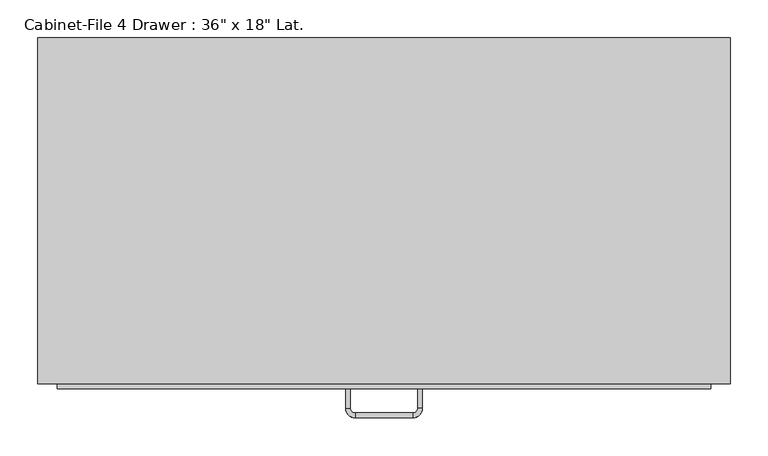
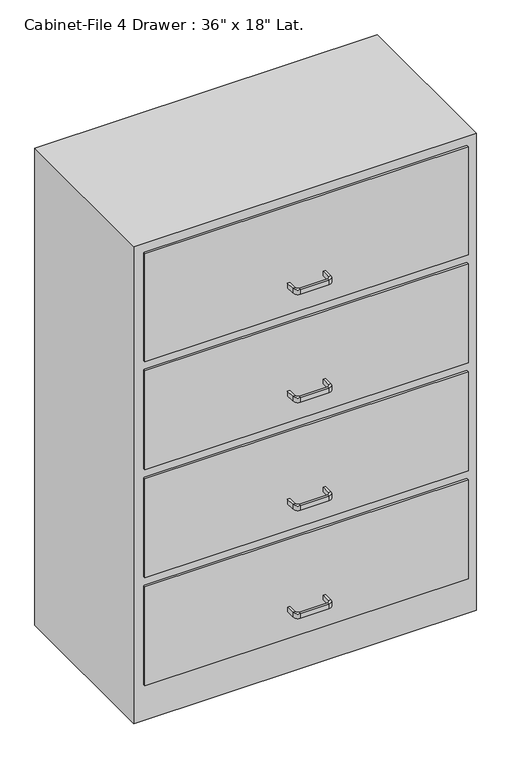
"""IFC4 building model written with IfcOpenShell, lengths in millimetres: furniture geometry."""

from ifc_helpers import new_model, si_unit, frame, origin, origin_with_axes, place, context, project, spatial, polyline, circle_curve, outline, extrude, source, transform, mapped, element, save
from ifc_brep_helpers import plane_surface, cylinder_surface, revolved_surface, advanced_brep


def furniture_7033c86c(model_context):
    return source(origin(), model_context, "Body", "SolidModel", [
        extrude(outline(polyline([(329.303553, 86.4656999), (329.303553, -370.7343001), (-585.096447, -370.7343001), (-585.096447, 86.4656999), (329.303553, 86.4656999)])), origin_with_axes(), (0.0, 0.0, 1.0), 1346.2),
        extrude(outline(polyline([(303.903553, -377.0843001), (-559.696447, -377.0843001), (-559.696447, -370.7343001), (303.903553, -370.7343001), (303.903553, -377.0843001)])), frame((0.0, 0.0, 1016.0), z_axis=(0.0, 0.0, 1.0), x_axis=(1.0, 0.0, 0.0)), (0.0, 0.0, 1.0), 304.8),
        extrude(outline(polyline([(303.903553, -377.0843001), (-559.696447, -377.0843001), (-559.696447, -370.7343001), (303.903553, -370.7343001), (303.903553, -377.0843001)])), frame((0.0, 0.0, 711.2), z_axis=(0.0, 0.0, 1.0), x_axis=(1.0, 0.0, 0.0)), (0.0, 0.0, 1.0), 279.4),
        extrude(outline(polyline([(303.903553, -377.0843001), (-559.696447, -377.0843001), (-559.696447, -370.7343001), (303.903553, -370.7343001), (303.903553, -377.0843001)])), frame((0.0, 0.0, 406.4), z_axis=(0.0, 0.0, 1.0), x_axis=(1.0, 0.0, 0.0)), (0.0, 0.0, 1.0), 279.4),
        extrude(outline(polyline([(303.903553, -377.0843001), (-559.696447, -377.0843001), (-559.696447, -370.7343001), (303.903553, -370.7343001), (303.903553, -377.0843001)])), frame((0.0, 0.0, 101.6), z_axis=(0.0, 0.0, 1.0), x_axis=(1.0, 0.0, 0.0)), (0.0, 0.0, 1.0), 279.4),
        advanced_brep(
        [(-172.346447, -377.0843001, 177.8), (-178.696447, -377.0843001, 177.8), (-178.696447, -377.0843001, 190.5), (-172.346447, -377.0843001, 190.5), (-172.346447, -402.4843001, 177.8), (-178.696447, -402.4843001, 177.8), (-178.696447, -402.4843001, 190.5), (-172.346447, -402.4843001, 190.5), (-165.996447, -415.1843001, 177.8), (-165.996447, -408.8343001, 177.8), (-165.996447, -415.1843001, 190.5), (-165.996447, -408.8343001, 190.5), (-89.796447, -408.8343001, 177.8), (-89.796447, -415.1843001, 177.8), (-89.796447, -415.1843001, 190.5), (-89.796447, -408.8343001, 190.5), (-77.096447, -402.4843001, 177.8), (-83.446447, -402.4843001, 177.8), (-77.096447, -402.4843001, 190.5), (-83.446447, -402.4843001, 190.5), (-83.446447, -377.0843001, 177.8), (-83.446447, -377.0843001, 190.5), (-77.096447, -377.0843001, 190.5), (-77.096447, -377.0843001, 177.8)],
        [
            (0, 1),
            (1, 2),
            (2, 3),
            (3, 0),
            (0, 4),
            (4, 5),
            (5, 1),
            (5, 6),
            (6, 2),
            (6, 7),
            (7, 3),
            (7, 4),
            (8, 5, circle_curve(frame((-165.996447, -402.4843001, 177.8), z_axis=(0.0, 0.0, -1.0), x_axis=(-1.0, 0.0, 0.0)), 12.7)),
            (4, 9, circle_curve(frame((-165.996447, -402.4843001, 177.8), z_axis=(0.0, 0.0, 1.0), x_axis=(-1.0, 0.0, 0.0)), 6.35)),
            (9, 8),
            (10, 6, circle_curve(frame((-165.996447, -402.4843001, 190.5), z_axis=(0.0, 0.0, -1.0), x_axis=(-1.0, 0.0, 0.0)), 12.7)),
            (8, 10),
            (11, 7, circle_curve(frame((-165.996447, -402.4843001, 190.5), z_axis=(0.0, 0.0, -1.0), x_axis=(-1.0, 0.0, 0.0)), 6.35)),
            (10, 11),
            (11, 9),
            (9, 12),
            (12, 13),
            (13, 8),
            (13, 14),
            (14, 10),
            (14, 15),
            (15, 11),
            (15, 12),
            (16, 13, circle_curve(frame((-89.796447, -402.4843001, 177.8), z_axis=(0.0, 0.0, -1.0), x_axis=(0.0, -1.0, 0.0)), 12.7)),
            (12, 17, circle_curve(frame((-89.796447, -402.4843001, 177.8), z_axis=(0.0, 0.0, 1.0), x_axis=(0.0, -1.0, 0.0)), 6.35)),
            (17, 16),
            (18, 14, circle_curve(frame((-89.796447, -402.4843001, 190.5), z_axis=(0.0, 0.0, -1.0), x_axis=(0.0, -1.0, 0.0)), 12.7)),
            (16, 18),
            (19, 15, circle_curve(frame((-89.796447, -402.4843001, 190.5), z_axis=(0.0, 0.0, -1.0), x_axis=(0.0, -1.0, 0.0)), 6.35)),
            (18, 19),
            (19, 17),
            (20, 21),
            (21, 22),
            (22, 23),
            (23, 20),
            (17, 20),
            (23, 16),
            (22, 18),
            (21, 19),
        ],
        [
            plane_surface(frame((-1283.614694, -377.0843001, 0.0), z_axis=(0.0, 1.0, 0.0), x_axis=(0.0, 0.0, -1.0))),
            plane_surface(frame((-172.346447, -377.0843001, 177.8), z_axis=(0.0, 0.0, -1.0), x_axis=(0.0, -1.0, 0.0))),
            plane_surface(frame((-178.696447, -377.0843001, 177.8), z_axis=(-1.0, 0.0, 0.0), x_axis=(0.0, -1.0, 0.0))),
            plane_surface(frame((-178.696447, -377.0843001, 190.5), z_axis=(0.0, 0.0, 1.0), x_axis=(0.0, -1.0, 0.0))),
            plane_surface(frame((-172.346447, -377.0843001, 190.5), z_axis=(1.0, 0.0, 0.0), x_axis=(0.0, -1.0, 0.0))),
            plane_surface(frame((-165.996447, -402.4843001, 177.8), z_axis=(0.0, 0.0, -1.0), x_axis=(-1.0, 0.0, 0.0))),
            cylinder_surface(frame((-165.996447, -402.4843001, 0.0), z_axis=(0.0, 0.0, 1.0), x_axis=(-1.0, 0.0, 0.0)), 12.7),
            plane_surface(frame((-165.996447, -402.4843001, 190.5), z_axis=(0.0, 0.0, 1.0), x_axis=(-1.0, 0.0, 0.0))),
            revolved_surface(polyline([(-172.34644699999998, -402.4843001, 190.5), (-172.34644699999998, -402.4843001, 177.8)]), (-165.996447, -402.4843001, 0.0), (0.0, 0.0, 1.0)),
            plane_surface(frame((-165.996447, -408.8343001, 177.8), z_axis=(0.0, 0.0, -1.0), x_axis=(1.0, 0.0, 0.0))),
            plane_surface(frame((-165.996447, -415.1843001, 177.8), z_axis=(0.0, -1.0, 0.0), x_axis=(1.0, 0.0, 0.0))),
            plane_surface(frame((-165.996447, -415.1843001, 190.5), z_axis=(0.0, 0.0, 1.0), x_axis=(1.0, 0.0, 0.0))),
            plane_surface(frame((-165.996447, -408.8343001, 190.5), z_axis=(0.0, 1.0, 0.0), x_axis=(1.0, 0.0, 0.0))),
            plane_surface(frame((-89.796447, -402.4843001, 177.8), z_axis=(0.0, 0.0, -1.0), x_axis=(0.0, -1.0, 0.0))),
            cylinder_surface(frame((-89.796447, -402.4843001, 0.0), z_axis=(0.0, 0.0, 1.0), x_axis=(0.0, -1.0, 0.0)), 12.7),
            plane_surface(frame((-89.796447, -402.4843001, 190.5), z_axis=(0.0, 0.0, 1.0), x_axis=(0.0, -1.0, 0.0))),
            revolved_surface(polyline([(-89.796447, -408.8343001, 190.5), (-89.796447, -408.8343001, 177.8)]), (-89.796447, -402.4843001, 0.0), (0.0, 0.0, 1.0)),
            plane_surface(frame((-1182.014694, -377.0843001, 0.0), z_axis=(0.0, 1.0, 0.0), x_axis=(0.0, 0.0, 1.0))),
            plane_surface(frame((-83.446447, -402.4843001, 177.8), z_axis=(0.0, 0.0, -1.0), x_axis=(0.0, 1.0, 0.0))),
            plane_surface(frame((-77.096447, -402.4843001, 177.8), z_axis=(1.0, 0.0, 0.0), x_axis=(0.0, 1.0, 0.0))),
            plane_surface(frame((-77.096447, -402.4843001, 190.5), z_axis=(0.0, 0.0, 1.0), x_axis=(0.0, 1.0, 0.0))),
            plane_surface(frame((-83.446447, -402.4843001, 190.5), z_axis=(-1.0, 0.0, 0.0), x_axis=(0.0, 1.0, 0.0))),
        ],
        [
            (0, [[1, 2, 3, 4]]),
            (1, [[-1, 5, 6, 7]]),
            (2, [[-2, -7, 8, 9]]),
            (3, [[-3, -9, 10, 11]]),
            (4, [[-4, -11, 12, -5]]),
            (5, [[13, -6, 14, 15]]),
            (6, [[16, -8, -13, 17]]),
            (7, [[18, -10, -16, 19]]),
            (8, [[-14, -12, -18, 20]]),
            (9, [[-15, 21, 22, 23]]),
            (10, [[-17, -23, 24, 25]]),
            (11, [[-19, -25, 26, 27]]),
            (12, [[-20, -27, 28, -21]]),
            (13, [[29, -22, 30, 31]]),
            (14, [[32, -24, -29, 33]]),
            (15, [[34, -26, -32, 35]]),
            (16, [[-30, -28, -34, 36]]),
            (17, [[37, 38, 39, 40]]),
            (18, [[-31, 41, -40, 42]]),
            (19, [[-33, -42, -39, 43]]),
            (20, [[-35, -43, -38, 44]]),
            (21, [[-36, -44, -37, -41]]),
        ],
    ),
        advanced_brep(
        [(-172.346447, -377.0843001, 482.6), (-178.696447, -377.0843001, 482.6), (-178.696447, -377.0843001, 495.3), (-172.346447, -377.0843001, 495.3), (-172.346447, -402.4843001, 482.6), (-178.696447, -402.4843001, 482.6), (-178.696447, -402.4843001, 495.3), (-172.346447, -402.4843001, 495.3), (-165.996447, -415.1843001, 482.6), (-165.996447, -408.8343001, 482.6), (-165.996447, -415.1843001, 495.3), (-165.996447, -408.8343001, 495.3), (-89.796447, -408.8343001, 482.6), (-89.796447, -415.1843001, 482.6), (-89.796447, -415.1843001, 495.3), (-89.796447, -408.8343001, 495.3), (-77.096447, -402.4843001, 482.6), (-83.446447, -402.4843001, 482.6), (-77.096447, -402.4843001, 495.3), (-83.446447, -402.4843001, 495.3), (-83.446447, -377.0843001, 482.6), (-83.446447, -377.0843001, 495.3), (-77.096447, -377.0843001, 495.3), (-77.096447, -377.0843001, 482.6)],
        [
            (0, 1),
            (1, 2),
            (2, 3),
            (3, 0),
            (0, 4),
            (4, 5),
            (5, 1),
            (5, 6),
            (6, 2),
            (6, 7),
            (7, 3),
            (7, 4),
            (8, 5, circle_curve(frame((-165.996447, -402.4843001, 482.6), z_axis=(0.0, 0.0, -1.0), x_axis=(-1.0, 0.0, 0.0)), 12.7)),
            (4, 9, circle_curve(frame((-165.996447, -402.4843001, 482.6), z_axis=(0.0, 0.0, 1.0), x_axis=(-1.0, 0.0, 0.0)), 6.35)),
            (9, 8),
            (10, 6, circle_curve(frame((-165.996447, -402.4843001, 495.3), z_axis=(0.0, 0.0, -1.0), x_axis=(-1.0, 0.0, 0.0)), 12.7)),
            (8, 10),
            (11, 7, circle_curve(frame((-165.996447, -402.4843001, 495.3), z_axis=(0.0, 0.0, -1.0), x_axis=(-1.0, 0.0, 0.0)), 6.35)),
            (10, 11),
            (11, 9),
            (9, 12),
            (12, 13),
            (13, 8),
            (13, 14),
            (14, 10),
            (14, 15),
            (15, 11),
            (15, 12),
            (16, 13, circle_curve(frame((-89.796447, -402.4843001, 482.6), z_axis=(0.0, 0.0, -1.0), x_axis=(0.0, -1.0, 0.0)), 12.7)),
            (12, 17, circle_curve(frame((-89.796447, -402.4843001, 482.6), z_axis=(0.0, 0.0, 1.0), x_axis=(0.0, -1.0, 0.0)), 6.35)),
            (17, 16),
            (18, 14, circle_curve(frame((-89.796447, -402.4843001, 495.3), z_axis=(0.0, 0.0, -1.0), x_axis=(0.0, -1.0, 0.0)), 12.7)),
            (16, 18),
            (19, 15, circle_curve(frame((-89.796447, -402.4843001, 495.3), z_axis=(0.0, 0.0, -1.0), x_axis=(0.0, -1.0, 0.0)), 6.35)),
            (18, 19),
            (19, 17),
            (20, 21),
            (21, 22),
            (22, 23),
            (23, 20),
            (17, 20),
            (23, 16),
            (22, 18),
            (21, 19),
        ],
        [
            plane_surface(frame((-1283.614694, -377.0843001, 0.0), z_axis=(0.0, 1.0, 0.0), x_axis=(0.0, 0.0, -1.0))),
            plane_surface(frame((-172.346447, -377.0843001, 482.6), z_axis=(0.0, 0.0, -1.0), x_axis=(0.0, -1.0, 0.0))),
            plane_surface(frame((-178.696447, -377.0843001, 482.6), z_axis=(-1.0, 0.0, 0.0), x_axis=(0.0, -1.0, 0.0))),
            plane_surface(frame((-178.696447, -377.0843001, 495.3), z_axis=(0.0, 0.0, 1.0), x_axis=(0.0, -1.0, 0.0))),
            plane_surface(frame((-172.346447, -377.0843001, 495.3), z_axis=(1.0, 0.0, 0.0), x_axis=(0.0, -1.0, 0.0))),
            plane_surface(frame((-165.996447, -402.4843001, 482.6), z_axis=(0.0, 0.0, -1.0), x_axis=(-1.0, 0.0, 0.0))),
            cylinder_surface(frame((-165.996447, -402.4843001, 0.0), z_axis=(0.0, 0.0, 1.0), x_axis=(-1.0, 0.0, 0.0)), 12.7),
            plane_surface(frame((-165.996447, -402.4843001, 495.3), z_axis=(0.0, 0.0, 1.0), x_axis=(-1.0, 0.0, 0.0))),
            revolved_surface(polyline([(-172.34644699999998, -402.4843001, 495.3), (-172.34644699999998, -402.4843001, 482.6)]), (-165.996447, -402.4843001, 0.0), (0.0, 0.0, 1.0)),
            plane_surface(frame((-165.996447, -408.8343001, 482.6), z_axis=(0.0, 0.0, -1.0), x_axis=(1.0, 0.0, 0.0))),
            plane_surface(frame((-165.996447, -415.1843001, 482.6), z_axis=(0.0, -1.0, 0.0), x_axis=(1.0, 0.0, 0.0))),
            plane_surface(frame((-165.996447, -415.1843001, 495.3), z_axis=(0.0, 0.0, 1.0), x_axis=(1.0, 0.0, 0.0))),
            plane_surface(frame((-165.996447, -408.8343001, 495.3), z_axis=(0.0, 1.0, 0.0), x_axis=(1.0, 0.0, 0.0))),
            plane_surface(frame((-89.796447, -402.4843001, 482.6), z_axis=(0.0, 0.0, -1.0), x_axis=(0.0, -1.0, 0.0))),
            cylinder_surface(frame((-89.796447, -402.4843001, 0.0), z_axis=(0.0, 0.0, 1.0), x_axis=(0.0, -1.0, 0.0)), 12.7),
            plane_surface(frame((-89.796447, -402.4843001, 495.3), z_axis=(0.0, 0.0, 1.0), x_axis=(0.0, -1.0, 0.0))),
            revolved_surface(polyline([(-89.796447, -408.8343001, 495.3), (-89.796447, -408.8343001, 482.6)]), (-89.796447, -402.4843001, 0.0), (0.0, 0.0, 1.0)),
            plane_surface(frame((-1182.014694, -377.0843001, 0.0), z_axis=(0.0, 1.0, 0.0), x_axis=(0.0, 0.0, 1.0))),
            plane_surface(frame((-83.446447, -402.4843001, 482.6), z_axis=(0.0, 0.0, -1.0), x_axis=(0.0, 1.0, 0.0))),
            plane_surface(frame((-77.096447, -402.4843001, 482.6), z_axis=(1.0, 0.0, 0.0), x_axis=(0.0, 1.0, 0.0))),
            plane_surface(frame((-77.096447, -402.4843001, 495.3), z_axis=(0.0, 0.0, 1.0), x_axis=(0.0, 1.0, 0.0))),
            plane_surface(frame((-83.446447, -402.4843001, 495.3), z_axis=(-1.0, 0.0, 0.0), x_axis=(0.0, 1.0, 0.0))),
        ],
        [
            (0, [[1, 2, 3, 4]]),
            (1, [[-1, 5, 6, 7]]),
            (2, [[-2, -7, 8, 9]]),
            (3, [[-3, -9, 10, 11]]),
            (4, [[-4, -11, 12, -5]]),
            (5, [[13, -6, 14, 15]]),
            (6, [[16, -8, -13, 17]]),
            (7, [[18, -10, -16, 19]]),
            (8, [[-14, -12, -18, 20]]),
            (9, [[-15, 21, 22, 23]]),
            (10, [[-17, -23, 24, 25]]),
            (11, [[-19, -25, 26, 27]]),
            (12, [[-20, -27, 28, -21]]),
            (13, [[29, -22, 30, 31]]),
            (14, [[32, -24, -29, 33]]),
            (15, [[34, -26, -32, 35]]),
            (16, [[-30, -28, -34, 36]]),
            (17, [[37, 38, 39, 40]]),
            (18, [[-31, 41, -40, 42]]),
            (19, [[-33, -42, -39, 43]]),
            (20, [[-35, -43, -38, 44]]),
            (21, [[-36, -44, -37, -41]]),
        ],
    ),
        advanced_brep(
        [(-172.346447, -377.0843001, 787.4), (-178.696447, -377.0843001, 787.4), (-178.696447, -377.0843001, 800.1), (-172.346447, -377.0843001, 800.1), (-172.346447, -402.4843001, 787.4), (-178.696447, -402.4843001, 787.4), (-178.696447, -402.4843001, 800.1), (-172.346447, -402.4843001, 800.1), (-165.996447, -415.1843001, 787.4), (-165.996447, -408.8343001, 787.4), (-165.996447, -415.1843001, 800.1), (-165.996447, -408.8343001, 800.1), (-89.796447, -408.8343001, 787.4), (-89.796447, -415.1843001, 787.4), (-89.796447, -415.1843001, 800.1), (-89.796447, -408.8343001, 800.1), (-77.096447, -402.4843001, 787.4), (-83.446447, -402.4843001, 787.4), (-77.096447, -402.4843001, 800.1), (-83.446447, -402.4843001, 800.1), (-83.446447, -377.0843001, 787.4), (-83.446447, -377.0843001, 800.1), (-77.096447, -377.0843001, 800.1), (-77.096447, -377.0843001, 787.4)],
        [
            (0, 1),
            (1, 2),
            (2, 3),
            (3, 0),
            (0, 4),
            (4, 5),
            (5, 1),
            (5, 6),
            (6, 2),
            (6, 7),
            (7, 3),
            (7, 4),
            (8, 5, circle_curve(frame((-165.996447, -402.4843001, 787.4), z_axis=(0.0, 0.0, -1.0), x_axis=(-1.0, 0.0, 0.0)), 12.7)),
            (4, 9, circle_curve(frame((-165.996447, -402.4843001, 787.4), z_axis=(0.0, 0.0, 1.0), x_axis=(-1.0, 0.0, 0.0)), 6.35)),
            (9, 8),
            (10, 6, circle_curve(frame((-165.996447, -402.4843001, 800.1), z_axis=(0.0, 0.0, -1.0), x_axis=(-1.0, 0.0, 0.0)), 12.7)),
            (8, 10),
            (11, 7, circle_curve(frame((-165.996447, -402.4843001, 800.1), z_axis=(0.0, 0.0, -1.0), x_axis=(-1.0, 0.0, 0.0)), 6.35)),
            (10, 11),
            (11, 9),
            (9, 12),
            (12, 13),
            (13, 8),
            (13, 14),
            (14, 10),
            (14, 15),
            (15, 11),
            (15, 12),
            (16, 13, circle_curve(frame((-89.796447, -402.4843001, 787.4), z_axis=(0.0, 0.0, -1.0), x_axis=(0.0, -1.0, 0.0)), 12.7)),
            (12, 17, circle_curve(frame((-89.796447, -402.4843001, 787.4), z_axis=(0.0, 0.0, 1.0), x_axis=(0.0, -1.0, 0.0)), 6.35)),
            (17, 16),
            (18, 14, circle_curve(frame((-89.796447, -402.4843001, 800.1), z_axis=(0.0, 0.0, -1.0), x_axis=(0.0, -1.0, 0.0)), 12.7)),
            (16, 18),
            (19, 15, circle_curve(frame((-89.796447, -402.4843001, 800.1), z_axis=(0.0, 0.0, -1.0), x_axis=(0.0, -1.0, 0.0)), 6.35)),
            (18, 19),
            (19, 17),
            (20, 21),
            (21, 22),
            (22, 23),
            (23, 20),
            (17, 20),
            (23, 16),
            (22, 18),
            (21, 19),
        ],
        [
            plane_surface(frame((-1283.614694, -377.0843001, 0.0), z_axis=(0.0, 1.0, 0.0), x_axis=(0.0, 0.0, -1.0))),
            plane_surface(frame((-172.346447, -377.0843001, 787.4), z_axis=(0.0, 0.0, -1.0), x_axis=(0.0, -1.0, 0.0))),
            plane_surface(frame((-178.696447, -377.0843001, 787.4), z_axis=(-1.0, 0.0, 0.0), x_axis=(0.0, -1.0, 0.0))),
            plane_surface(frame((-178.696447, -377.0843001, 800.1), z_axis=(0.0, 0.0, 1.0), x_axis=(0.0, -1.0, 0.0))),
            plane_surface(frame((-172.346447, -377.0843001, 800.1), z_axis=(1.0, 0.0, 0.0), x_axis=(0.0, -1.0, 0.0))),
            plane_surface(frame((-165.996447, -402.4843001, 787.4), z_axis=(0.0, 0.0, -1.0), x_axis=(-1.0, 0.0, 0.0))),
            cylinder_surface(frame((-165.996447, -402.4843001, 0.0), z_axis=(0.0, 0.0, 1.0), x_axis=(-1.0, 0.0, 0.0)), 12.7),
            plane_surface(frame((-165.996447, -402.4843001, 800.1), z_axis=(0.0, 0.0, 1.0), x_axis=(-1.0, 0.0, 0.0))),
            revolved_surface(polyline([(-172.34644699999998, -402.4843001, 800.1), (-172.34644699999998, -402.4843001, 787.4)]), (-165.996447, -402.4843001, 0.0), (0.0, 0.0, 1.0)),
            plane_surface(frame((-165.996447, -408.8343001, 787.4), z_axis=(0.0, 0.0, -1.0), x_axis=(1.0, 0.0, 0.0))),
            plane_surface(frame((-165.996447, -415.1843001, 787.4), z_axis=(0.0, -1.0, 0.0), x_axis=(1.0, 0.0, 0.0))),
            plane_surface(frame((-165.996447, -415.1843001, 800.1), z_axis=(0.0, 0.0, 1.0), x_axis=(1.0, 0.0, 0.0))),
            plane_surface(frame((-165.996447, -408.8343001, 800.1), z_axis=(0.0, 1.0, 0.0), x_axis=(1.0, 0.0, 0.0))),
            plane_surface(frame((-89.796447, -402.4843001, 787.4), z_axis=(0.0, 0.0, -1.0), x_axis=(0.0, -1.0, 0.0))),
            cylinder_surface(frame((-89.796447, -402.4843001, 0.0), z_axis=(0.0, 0.0, 1.0), x_axis=(0.0, -1.0, 0.0)), 12.7),
            plane_surface(frame((-89.796447, -402.4843001, 800.1), z_axis=(0.0, 0.0, 1.0), x_axis=(0.0, -1.0, 0.0))),
            revolved_surface(polyline([(-89.796447, -408.8343001, 800.1), (-89.796447, -408.8343001, 787.4)]), (-89.796447, -402.4843001, 0.0), (0.0, 0.0, 1.0)),
            plane_surface(frame((-1182.014694, -377.0843001, 0.0), z_axis=(0.0, 1.0, 0.0), x_axis=(0.0, 0.0, 1.0))),
            plane_surface(frame((-83.446447, -402.4843001, 787.4), z_axis=(0.0, 0.0, -1.0), x_axis=(0.0, 1.0, 0.0))),
            plane_surface(frame((-77.096447, -402.4843001, 787.4), z_axis=(1.0, 0.0, 0.0), x_axis=(0.0, 1.0, 0.0))),
            plane_surface(frame((-77.096447, -402.4843001, 800.1), z_axis=(0.0, 0.0, 1.0), x_axis=(0.0, 1.0, 0.0))),
            plane_surface(frame((-83.446447, -402.4843001, 800.1), z_axis=(-1.0, 0.0, 0.0), x_axis=(0.0, 1.0, 0.0))),
        ],
        [
            (0, [[1, 2, 3, 4]]),
            (1, [[-1, 5, 6, 7]]),
            (2, [[-2, -7, 8, 9]]),
            (3, [[-3, -9, 10, 11]]),
            (4, [[-4, -11, 12, -5]]),
            (5, [[13, -6, 14, 15]]),
            (6, [[16, -8, -13, 17]]),
            (7, [[18, -10, -16, 19]]),
            (8, [[-14, -12, -18, 20]]),
            (9, [[-15, 21, 22, 23]]),
            (10, [[-17, -23, 24, 25]]),
            (11, [[-19, -25, 26, 27]]),
            (12, [[-20, -27, 28, -21]]),
            (13, [[29, -22, 30, 31]]),
            (14, [[32, -24, -29, 33]]),
            (15, [[34, -26, -32, 35]]),
            (16, [[-30, -28, -34, 36]]),
            (17, [[37, 38, 39, 40]]),
            (18, [[-31, 41, -40, 42]]),
            (19, [[-33, -42, -39, 43]]),
            (20, [[-35, -43, -38, 44]]),
            (21, [[-36, -44, -37, -41]]),
        ],
    ),
        advanced_brep(
        [(-172.346447, -377.0843001, 1092.2), (-178.696447, -377.0843001, 1092.2), (-178.696447, -377.0843001, 1104.9), (-172.346447, -377.0843001, 1104.9), (-172.346447, -402.4843001, 1092.2), (-178.696447, -402.4843001, 1092.2), (-178.696447, -402.4843001, 1104.9), (-172.346447, -402.4843001, 1104.9), (-165.996447, -415.1843001, 1092.2), (-165.996447, -408.8343001, 1092.2), (-165.996447, -415.1843001, 1104.9), (-165.996447, -408.8343001, 1104.9), (-89.796447, -408.8343001, 1092.2), (-89.796447, -415.1843001, 1092.2), (-89.796447, -415.1843001, 1104.9), (-89.796447, -408.8343001, 1104.9), (-77.096447, -402.4843001, 1092.2), (-83.446447, -402.4843001, 1092.2), (-77.096447, -402.4843001, 1104.9), (-83.446447, -402.4843001, 1104.9), (-83.446447, -377.0843001, 1092.2), (-83.446447, -377.0843001, 1104.9), (-77.096447, -377.0843001, 1104.9), (-77.096447, -377.0843001, 1092.2)],
        [
            (0, 1),
            (1, 2),
            (2, 3),
            (3, 0),
            (0, 4),
            (4, 5),
            (5, 1),
            (5, 6),
            (6, 2),
            (6, 7),
            (7, 3),
            (7, 4),
            (8, 5, circle_curve(frame((-165.996447, -402.4843001, 1092.2), z_axis=(0.0, 0.0, -1.0), x_axis=(-1.0, 0.0, 0.0)), 12.7)),
            (4, 9, circle_curve(frame((-165.996447, -402.4843001, 1092.2), z_axis=(0.0, 0.0, 1.0), x_axis=(-1.0, 0.0, 0.0)), 6.35)),
            (9, 8),
            (10, 6, circle_curve(frame((-165.996447, -402.4843001, 1104.9), z_axis=(0.0, 0.0, -1.0), x_axis=(-1.0, 0.0, 0.0)), 12.7)),
            (8, 10),
            (11, 7, circle_curve(frame((-165.996447, -402.4843001, 1104.9), z_axis=(0.0, 0.0, -1.0), x_axis=(-1.0, 0.0, 0.0)), 6.35)),
            (10, 11),
            (11, 9),
            (9, 12),
            (12, 13),
            (13, 8),
            (13, 14),
            (14, 10),
            (14, 15),
            (15, 11),
            (15, 12),
            (16, 13, circle_curve(frame((-89.796447, -402.4843001, 1092.2), z_axis=(0.0, 0.0, -1.0), x_axis=(0.0, -1.0, 0.0)), 12.7)),
            (12, 17, circle_curve(frame((-89.796447, -402.4843001, 1092.2), z_axis=(0.0, 0.0, 1.0), x_axis=(0.0, -1.0, 0.0)), 6.35)),
            (17, 16),
            (18, 14, circle_curve(frame((-89.796447, -402.4843001, 1104.9), z_axis=(0.0, 0.0, -1.0), x_axis=(0.0, -1.0, 0.0)), 12.7)),
            (16, 18),
            (19, 15, circle_curve(frame((-89.796447, -402.4843001, 1104.9), z_axis=(0.0, 0.0, -1.0), x_axis=(0.0, -1.0, 0.0)), 6.35)),
            (18, 19),
            (19, 17),
            (20, 21),
            (21, 22),
            (22, 23),
            (23, 20),
            (17, 20),
            (23, 16),
            (22, 18),
            (21, 19),
        ],
        [
            plane_surface(frame((-1283.614694, -377.0843001, 0.0), z_axis=(0.0, 1.0, 0.0), x_axis=(0.0, 0.0, -1.0))),
            plane_surface(frame((-172.346447, -377.0843001, 1092.2), z_axis=(0.0, 0.0, -1.0), x_axis=(0.0, -1.0, 0.0))),
            plane_surface(frame((-178.696447, -377.0843001, 1092.2), z_axis=(-1.0, 0.0, 0.0), x_axis=(0.0, -1.0, 0.0))),
            plane_surface(frame((-178.696447, -377.0843001, 1104.9), z_axis=(0.0, 0.0, 1.0), x_axis=(0.0, -1.0, 0.0))),
            plane_surface(frame((-172.346447, -377.0843001, 1104.9), z_axis=(1.0, 0.0, 0.0), x_axis=(0.0, -1.0, 0.0))),
            plane_surface(frame((-165.996447, -402.4843001, 1092.2), z_axis=(0.0, 0.0, -1.0), x_axis=(-1.0, 0.0, 0.0))),
            cylinder_surface(frame((-165.996447, -402.4843001, 0.0), z_axis=(0.0, 0.0, 1.0), x_axis=(-1.0, 0.0, 0.0)), 12.7),
            plane_surface(frame((-165.996447, -402.4843001, 1104.9), z_axis=(0.0, 0.0, 1.0), x_axis=(-1.0, 0.0, 0.0))),
            revolved_surface(polyline([(-172.34644699999998, -402.4843001, 1104.9), (-172.34644699999998, -402.4843001, 1092.2)]), (-165.996447, -402.4843001, 0.0), (0.0, 0.0, 1.0)),
            plane_surface(frame((-165.996447, -408.8343001, 1092.2), z_axis=(0.0, 0.0, -1.0), x_axis=(1.0, 0.0, 0.0))),
            plane_surface(frame((-165.996447, -415.1843001, 1092.2), z_axis=(0.0, -1.0, 0.0), x_axis=(1.0, 0.0, 0.0))),
            plane_surface(frame((-165.996447, -415.1843001, 1104.9), z_axis=(0.0, 0.0, 1.0), x_axis=(1.0, 0.0, 0.0))),
            plane_surface(frame((-165.996447, -408.8343001, 1104.9), z_axis=(0.0, 1.0, 0.0), x_axis=(1.0, 0.0, 0.0))),
            plane_surface(frame((-89.796447, -402.4843001, 1092.2), z_axis=(0.0, 0.0, -1.0), x_axis=(0.0, -1.0, 0.0))),
            cylinder_surface(frame((-89.796447, -402.4843001, 0.0), z_axis=(0.0, 0.0, 1.0), x_axis=(0.0, -1.0, 0.0)), 12.7),
            plane_surface(frame((-89.796447, -402.4843001, 1104.9), z_axis=(0.0, 0.0, 1.0), x_axis=(0.0, -1.0, 0.0))),
            revolved_surface(polyline([(-89.796447, -408.8343001, 1104.9), (-89.796447, -408.8343001, 1092.2)]), (-89.796447, -402.4843001, 0.0), (0.0, 0.0, 1.0)),
            plane_surface(frame((-1182.014694, -377.0843001, 0.0), z_axis=(0.0, 1.0, 0.0), x_axis=(0.0, 0.0, 1.0))),
            plane_surface(frame((-83.446447, -402.4843001, 1092.2), z_axis=(0.0, 0.0, -1.0), x_axis=(0.0, 1.0, 0.0))),
            plane_surface(frame((-77.096447, -402.4843001, 1092.2), z_axis=(1.0, 0.0, 0.0), x_axis=(0.0, 1.0, 0.0))),
            plane_surface(frame((-77.096447, -402.4843001, 1104.9), z_axis=(0.0, 0.0, 1.0), x_axis=(0.0, 1.0, 0.0))),
            plane_surface(frame((-83.446447, -402.4843001, 1104.9), z_axis=(-1.0, 0.0, 0.0), x_axis=(0.0, 1.0, 0.0))),
        ],
        [
            (0, [[1, 2, 3, 4]]),
            (1, [[-1, 5, 6, 7]]),
            (2, [[-2, -7, 8, 9]]),
            (3, [[-3, -9, 10, 11]]),
            (4, [[-4, -11, 12, -5]]),
            (5, [[13, -6, 14, 15]]),
            (6, [[16, -8, -13, 17]]),
            (7, [[18, -10, -16, 19]]),
            (8, [[-14, -12, -18, 20]]),
            (9, [[-15, 21, 22, 23]]),
            (10, [[-17, -23, 24, 25]]),
            (11, [[-19, -25, 26, 27]]),
            (12, [[-20, -27, 28, -21]]),
            (13, [[29, -22, 30, 31]]),
            (14, [[32, -24, -29, 33]]),
            (15, [[34, -26, -32, 35]]),
            (16, [[-30, -28, -34, 36]]),
            (17, [[37, 38, 39, 40]]),
            (18, [[-31, 41, -40, 42]]),
            (19, [[-33, -42, -39, 43]]),
            (20, [[-35, -43, -38, 44]]),
            (21, [[-36, -44, -37, -41]]),
        ],
    ),
    ])


if __name__ == "__main__":
    model = new_model("IFC4")
    model_context = context("Model", 3, world=origin())
    ifc_project = project(units=[si_unit("LENGTHUNIT", "METRE", prefix="MILLI")], contexts=[model_context])
    site = spatial("IfcSite", under=ifc_project)
    building = spatial("IfcBuilding", under=site)
    placement = place(None, origin())
    furniture_shape = furniture_7033c86c(model_context)
    element("IfcFurniture", 1, ObjectType="Cabinet-File 4 Drawer : 36\" x 18\" Lat.", at=placement, inside=building, context=model_context, shape_type="MappedRepresentation", body=[
        mapped(furniture_shape, transform((0.0, 0.0, 0.0), x_axis=(1.0, 0.0, 0.0), y_axis=(0.0, 1.0, 0.0), z_axis=(0.0, 0.0, 1.0))),
    ])
    save(model, "model.ifc")

# Revit data of these elements
# Type "Cabinet-File 4 Drawer : 36\" x 18\" Lat."
#   Assembly Code = "E2020200"
#   Depth = 1' - 6"
#   Height = 4' - 5"
#   Width = 3' - 0"
#   Cabinet Material = Steel, Paint Finish, Ivory, Glossy
#   Handle Material = Steel, Chrome Plated
#   Default Elevation = 0
# Element 1 (IfcFurniture, "Cabinet-File 4 Drawer : 36\" x 18\" Lat.")
#   Materials on its faces: "Steel, Chrome Plated", "Steel, Paint Finish, Ivory, Glossy"
# Materials
#   "Steel, Paint Finish, Ivory, Glossy": class "Metal", colour RGB 247 247 239, transparency 0, Description = "Steel, paint finish, ivory, glossy", Cost = 0
#   "Steel, Chrome Plated": class "Metal", colour RGB 17 17 17, transparency 0, Description = "Chromiuim plated steel", Cost = 0
